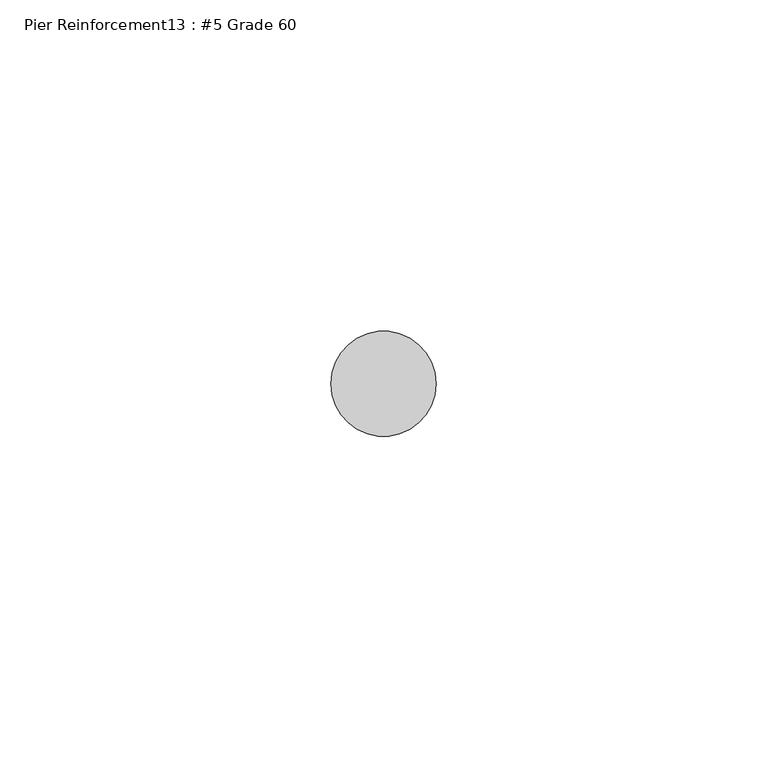
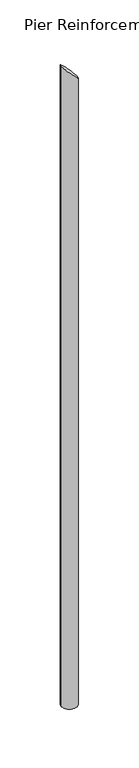
"""IFC4 building model written with IfcOpenShell, lengths in millimetres: proxy geometry, Pier Reinforcement13 : #5 Grade 60."""

import ifcopenshell
import ifcopenshell.guid

model = None  # the IFC model being written
_history = None  # IfcOwnerHistory: only IFC2X3 demands one
_inside = {}  # id of a spatial element -> (the spatial element, [elements in it])
_under = {}  # id of a project, library or spatial element -> (it, [spatial elements below it])
_declared = {}  # id of a project -> (the project, [libraries it declares])
_typed = {}  # id of a type object -> (the type object, [elements of that type])
_made_of = {}  # id of a material, layer set ... -> (it, [elements and type objects made of it])


def new_model(schema):
    """Start an empty IFC model of exactly this schema.

    Asked for "IFC4X3", IfcOpenShell would pick the latest addendum, in which some entities
    have other attributes; the version numbers below select the first issue.
    IFC2X3 requires an IfcOwnerHistory on every rooted entity: one is made here for all.
    """
    global model, _history
    if schema == "IFC4X3":
        model = ifcopenshell.file(schema_version=(4, 3, 0, 0))
    else:
        model = ifcopenshell.file(schema=schema)
    _inside.clear()
    _under.clear()
    _declared.clear()
    _typed.clear()
    _made_of.clear()
    _history = None
    if model.schema == "IFC2X3":
        org = make("IfcOrganization", Name="unknown")
        user = make(
            "IfcPersonAndOrganization",
            ThePerson=make("IfcPerson", FamilyName="unknown"),
            TheOrganization=org,
        )
        app = make(
            "IfcApplication",
            ApplicationDeveloper=org,
            Version="unknown",
            ApplicationFullName="unknown",
            ApplicationIdentifier="unknown",
        )
        _history = make(
            "IfcOwnerHistory",
            OwningUser=user,
            OwningApplication=app,
            ChangeAction="ADDED",
            CreationDate=0,
        )
    return model


def make(cls, **values):
    """One entity of the class cls with the attributes given. An attribute that is None is left unset."""
    return model.create_entity(
        cls, **{name: value for name, value in values.items() if value is not None}
    )


def rooted(cls, **values):
    """An entity with a GlobalId (a new one), such as an element, a storey or a relation."""
    return make(cls, GlobalId=ifcopenshell.guid.new(), OwnerHistory=_history, **values)


def si_unit(unit_type, name, prefix=None):
    """IfcSIUnit, for example si_unit("LENGTHUNIT", "METRE", prefix="MILLI")."""
    return make("IfcSIUnit", UnitType=unit_type, Prefix=prefix, Name=name)


def assignment(units):
    """IfcUnitAssignment: the units of a project."""
    return None if units is None else make("IfcUnitAssignment", Units=units)


def point(xyz):
    """IfcCartesianPoint."""
    return None if xyz is None else make("IfcCartesianPoint", Coordinates=xyz)


def direction(xyz):
    """IfcDirection."""
    return None if xyz is None else make("IfcDirection", DirectionRatios=xyz)


def frame(location, z_axis=None, x_axis=None):
    """IfcAxis2Placement3D, a coordinate frame: its origin and axes. An axis left out is left unset."""
    return make(
        "IfcAxis2Placement3D",
        Location=point(location),
        Axis=direction(z_axis),
        RefDirection=direction(x_axis),
    )


def origin():
    """The frame at (0, 0, 0) with its axes left unset."""
    return frame((0.0, 0.0, 0.0))


def place(relative_to, where):
    """IfcLocalPlacement: puts the frame where relative to a parent placement (None: the world)."""
    return make(
        "IfcLocalPlacement", PlacementRelTo=relative_to, RelativePlacement=where
    )


def context(
    kind, dimensions, precision=None, world=None, true_north=None, identifier=None
):
    """IfcGeometricRepresentationContext, for example the 3D "Model" context."""
    return make(
        "IfcGeometricRepresentationContext",
        ContextIdentifier=identifier,
        ContextType=kind,
        CoordinateSpaceDimension=dimensions,
        Precision=precision,
        WorldCoordinateSystem=world,
        TrueNorth=true_north,
    )


def project(units=None, contexts=None):
    """IfcProject with its units and contexts."""
    return rooted(
        "IfcProject",
        Name="project",
        RepresentationContexts=contexts,
        UnitsInContext=assignment(units),
    )


def spatial(cls, under=None, at=None, **own):
    """A site, building, storey or space (cls), placed at a placement, below another one or the project."""
    s = rooted(cls, ObjectPlacement=at, **own)
    if under is not None:
        _under.setdefault(under.id(), (under, []))[1].append(s)
    return s


def circle_curve(where, radius):
    """IfcCircle in the frame where."""
    return make("IfcCircle", Position=where, Radius=radius)


def ellipse_curve(where, semi_axis1, semi_axis2):
    """IfcEllipse in the frame where."""
    return make(
        "IfcEllipse", Position=where, SemiAxis1=semi_axis1, SemiAxis2=semi_axis2
    )


def shape(context_of_items, identifier, shape_type, items):
    """IfcShapeRepresentation: the items that make up one representation, for example the "Body"."""
    return make(
        "IfcShapeRepresentation",
        ContextOfItems=context_of_items,
        RepresentationIdentifier=identifier,
        RepresentationType=shape_type,
        Items=items,
    )


def source(mapping_origin, context_of_items, identifier, shape_type, items):
    """IfcRepresentationMap: a shape defined once, which mapped items show again and again."""
    return make(
        "IfcRepresentationMap",
        MappingOrigin=mapping_origin,
        MappedRepresentation=shape(context_of_items, identifier, shape_type, items),
    )


def transform(
    local_origin,
    x_axis=None,
    y_axis=None,
    z_axis=None,
    scale=None,
    scale2=None,
    scale3=None,
    uniform=True,
):
    """IfcCartesianTransformationOperator3D, or its non-uniform kind. x_axis, y_axis, z_axis: its Axis1, 2, 3."""
    if uniform:
        return make(
            "IfcCartesianTransformationOperator3D",
            Axis1=direction(x_axis),
            Axis2=direction(y_axis),
            LocalOrigin=point(local_origin),
            Scale=scale,
            Axis3=direction(z_axis),
        )
    return make(
        "IfcCartesianTransformationOperator3DnonUniform",
        Axis1=direction(x_axis),
        Axis2=direction(y_axis),
        LocalOrigin=point(local_origin),
        Scale=scale,
        Axis3=direction(z_axis),
        Scale2=scale2,
        Scale3=scale3,
    )


def mapped(mapping_source, mapping_target):
    """IfcMappedItem: shows the shape of a source again, moved by a transform."""
    return make(
        "IfcMappedItem", MappingSource=mapping_source, MappingTarget=mapping_target
    )


def made_of(thing, what):
    """Note that an element or type object is made of a material, layer set ...; save() writes the relation."""
    if what is not None:
        _made_of.setdefault(what.id(), (what, []))[1].append(thing)
    return thing


def element(
    cls,
    number,
    at=None,
    inside=None,
    cuts=None,
    type_object=None,
    material=None,
    context=None,
    identifier="Body",
    shape_type=None,
    held_by="IfcProductDefinitionShape",
    body=None,
    shapes=None,
    **own,
):
    """One element of the class cls, such as IfcWall. Its Tag is "e" and its number.

    at: its placement. inside: the storey or other place that contains it. cuts: it is an
    opening in that element (IfcRelVoidsElement). A single representation is given by context,
    identifier, shape_type and body (its items); several are given by shapes. held_by: the class
    of the entity that holds the representations. save() writes the other relations.
    """
    e = rooted(cls, Tag="e%d" % number, ObjectPlacement=at, **own)
    if body is not None:
        shapes = [shape(context, identifier, shape_type, body)]
    if shapes is not None:
        e.Representation = make(held_by, Representations=shapes)
    if inside is not None:
        _inside.setdefault(inside.id(), (inside, []))[1].append(e)
    if cuts is not None:
        rooted(
            "IfcRelVoidsElement", RelatingBuildingElement=cuts, RelatedOpeningElement=e
        )
    if type_object is not None:
        _typed.setdefault(type_object.id(), (type_object, []))[1].append(e)
    return made_of(e, material)


def aggregate(whole, parts):
    """IfcRelAggregates: a whole, such as a stair, and the parts it consists of."""
    return rooted("IfcRelAggregates", RelatingObject=whole, RelatedObjects=parts)


def save(model, path):
    """Write the relations noted so far, then the file.

    IfcRelAggregates (storeys below a building ...), IfcRelContainedInSpatialStructure (elements
    in a storey), IfcRelDefinesByType, IfcRelAssociatesMaterial and IfcRelDeclares: one each for
    every whole, place, type object, material and project.
    """
    for whole, parts in _under.values():
        aggregate(whole, parts)
    for where, things in _inside.values():
        rooted(
            "IfcRelContainedInSpatialStructure",
            RelatedElements=things,
            RelatingStructure=where,
        )
    for kind, things in _typed.values():
        rooted("IfcRelDefinesByType", RelatedObjects=things, RelatingType=kind)
    for what, things in _made_of.values():
        rooted("IfcRelAssociatesMaterial", RelatedObjects=things, RelatingMaterial=what)
    for by, libraries in _declared.values():
        rooted("IfcRelDeclares", RelatingContext=by, RelatedDefinitions=libraries)
    model.write(path)


def plane_surface(at):
    """IfcPlane: the flat surface through the origin of the frame at, square to its z axis."""
    return make("IfcPlane", Position=at)


def cylinder_surface(at, radius):
    """IfcCylindricalSurface: all points at the distance radius from the z axis of the frame at."""
    return make("IfcCylindricalSurface", Position=at, Radius=radius)


def advanced_brep(points, edges, surfaces, faces):
    """IfcAdvancedBrep: a solid bounded by faces that lie on surfaces and meet in shared edges.

    An edge is (start, end): straight between two places in points (the first is 0);
    or (start, end, curve); or (start, end, curve, False) where it runs against its curve.
    A face is (place in surfaces, loops), or (place, loops, False) where it looks against
    its surface's normal. A loop lists edges by number (the first is 1), with a minus sign
    where the edge is run from its end to its start. The first loop is the outer one.
    """
    corners = [point(p) for p in points]
    vertices = [make("IfcVertexPoint", VertexGeometry=c) for c in corners]
    made = []
    for start, end, *more in edges:
        made.append(
            make(
                "IfcEdgeCurve",
                EdgeStart=vertices[start],
                EdgeEnd=vertices[end],
                EdgeGeometry=more[0] if more else make("IfcPolyline", Points=[corners[start], corners[end]]),
                SameSense=more[1] if len(more) > 1 else True,
            )
        )
    hull = []
    for where, loops, *sense in faces:
        bounds = []
        for j, loop in enumerate(loops):
            ring = [make("IfcOrientedEdge", EdgeElement=made[abs(k) - 1], Orientation=k > 0) for k in loop]
            bounds.append(
                make(
                    "IfcFaceOuterBound" if j == 0 else "IfcFaceBound",
                    Bound=make("IfcEdgeLoop", EdgeList=ring),
                    Orientation=True,
                )
            )
        hull.append(make("IfcAdvancedFace", Bounds=bounds, FaceSurface=surfaces[where], SameSense=sense[0] if sense else True))
    return make("IfcAdvancedBrep", Outer=make("IfcClosedShell", CfsFaces=hull))


def pier_reinforcement13_5_grade_60_ff8834b7(model_context):
    return source(origin(), model_context, "Body", "AdvancedBrep", [
        advanced_brep(
        [(587484.5778122, -534096.6663841, -733.425), (587500.4528122, -534096.6663841, -733.425), (587500.4528122, -534096.6663841, -63.5), (587484.5778122, -534096.6663841, -47.625)],
        [
            (0, 1, circle_curve(frame((587492.5153122, -534096.6663841, -733.425), z_axis=(0.0, 0.0, -1.0), x_axis=(-1.0, 0.0, 0.0)), 7.9375)),
            (1, 0, circle_curve(frame((587492.5153122, -534096.6663841, -733.425), z_axis=(0.0, 0.0, -1.0), x_axis=(-1.0, 0.0, 0.0)), 7.9375)),
            (1, 2),
            (2, 3, ellipse_curve(frame((587492.5153122, -534096.6663841, -55.5625), z_axis=(-0.7071067811865458, 0.0, -0.7071067811865493), x_axis=(-0.7071067811865493, 0.0, 0.7071067811865456)), 11.2253202, 7.9375)),
            (3, 0),
            (3, 2, ellipse_curve(frame((587492.5153122, -534096.6663841, -55.5625), z_axis=(-0.7071067811865458, 0.0, -0.7071067811865493), x_axis=(-0.7071067811865493, 0.0, 0.7071067811865456)), 11.2253202, 7.9375)),
        ],
        [
            plane_surface(frame((587484.5778122, -534096.6663841, -733.425), z_axis=(0.0, 0.0, -1.0), x_axis=(0.0, 1.0, 0.0))),
            cylinder_surface(frame((587492.5153122, -534096.6663841, -733.425), z_axis=(0.0, 0.0, 1.0), x_axis=(-1.0, 0.0, 0.0)), 7.9375),
            plane_surface(frame((587484.5778122, -534071.2663841, -47.625), z_axis=(0.7071067811865458, 0.0, 0.7071067811865493), x_axis=(0.0, -1.0, 0.0))),
        ],
        [
            (0, [[1, 2]]),
            (1, [[-2, 3, 4, 5]]),
            (1, [[-1, -5, 6, -3]]),
            (2, [[-4, -6]]),
        ],
    ),
    ])


if __name__ == "__main__":
    model = new_model("IFC4")
    model_context = context("Model", 3, world=origin())
    ifc_project = project(units=[si_unit("LENGTHUNIT", "METRE", prefix="MILLI")], contexts=[model_context])
    site = spatial("IfcSite", under=ifc_project)
    building = spatial("IfcBuilding", under=site)
    placement = place(None, origin())
    pier_reinforcement13_5_grade_60_shape = pier_reinforcement13_5_grade_60_ff8834b7(model_context)
    element("IfcBuildingElementProxy", 1, Name="Pier Reinforcement13 : #5 Grade 60", ObjectType="Pier Reinforcement13 : #5 Grade 60", at=placement, inside=building, context=model_context, shape_type="MappedRepresentation", body=[
        mapped(pier_reinforcement13_5_grade_60_shape, transform((0.0, 0.0, 0.0), x_axis=(1.0, 0.0, 0.0), y_axis=(0.0, 1.0, 0.0), z_axis=(0.0, 0.0, 1.0))),
    ])
    save(model, "model.ifc")

# Revit data of these elements
# Element 1 (IfcBuildingElementProxy, "Pier Reinforcement13 : #5 Grade 60")
#   Materials on its faces: "#4 GR. 60 REINF. @ 16\" O.C. EW."
# Materials
#   "#4 GR. 60 REINF. @ 16\" O.C. EW.": class "Generic", colour RGB 84 83 81, transparency 0, Cost = 0
